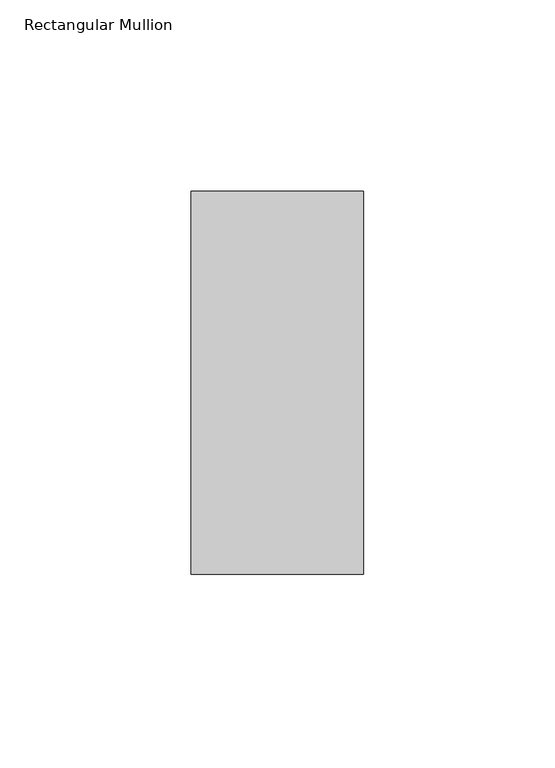
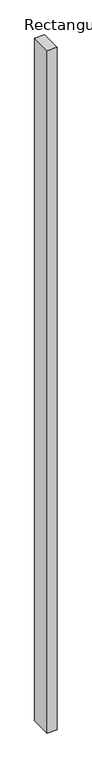
"""IFC4 building model written with IfcOpenShell, lengths in millimetres: member geometry, Rectangular Mullion : 알루미늄_Rectangular Cap_100 x 45."""

from ifc_helpers import new_model, si_unit, frame, origin, place, context, project, spatial, polyline, outline, extrude, source, transform, mapped, element, save


def rectangular_mullion_73c25319(model_context):
    return source(origin(), model_context, "Body", "SweptSolid", [
        extrude(outline(polyline([(0.0, 50.0), (0.0, -50.0), (-45.0, -50.0), (-45.0, 50.0), (0.0, 50.0)])), frame((0.0, 0.0, -3325.0), z_axis=(0.0, 0.0, 1.0), x_axis=(1.0, 0.0, 0.0)), (0.0, 0.0, 1.0), 3325.0),
    ])


if __name__ == "__main__":
    model = new_model("IFC4")
    model_context = context("Model", 3, world=origin())
    ifc_project = project(units=[si_unit("LENGTHUNIT", "METRE", prefix="MILLI")], contexts=[model_context])
    site = spatial("IfcSite", under=ifc_project)
    building = spatial("IfcBuilding", under=site)
    placement = place(None, origin())
    rectangular_mullion_shape = rectangular_mullion_73c25319(model_context)
    element("IfcMember", 1, ObjectType="Rectangular Mullion : 알루미늄_Rectangular Cap_100 x 45", at=placement, inside=building, context=model_context, shape_type="MappedRepresentation", body=[
        mapped(rectangular_mullion_shape, transform((0.0, 0.0, 0.0), x_axis=(1.0, 0.0, 0.0), y_axis=(0.0, 1.0, 0.0), z_axis=(0.0, 0.0, 1.0))),
    ])
    save(model, "model.ifc")

# Revit data of these elements
# Type "Rectangular Mullion : 알루미늄_Rectangular Cap_100 x 45"
#   built-in parameter 1007304 = 0.328084 (stored number, unit not read)
#   built-in parameter 1007301 = 0.0738189 (stored number, unit not read)
#   built-in parameter 1007300 = 0.0738189 (stored number, unit not read)
# Element 1 (IfcMember, "Rectangular Mullion : 알루미늄_Rectangular Cap_100 x 45")
#   Materials on its faces: "00_Metal_Stainless Steel"
# Materials
#   "00_Metal_Stainless Steel": class "Metal", colour RGB 148 148 148, transparency 0, Description = "Steel", Cost = 0
